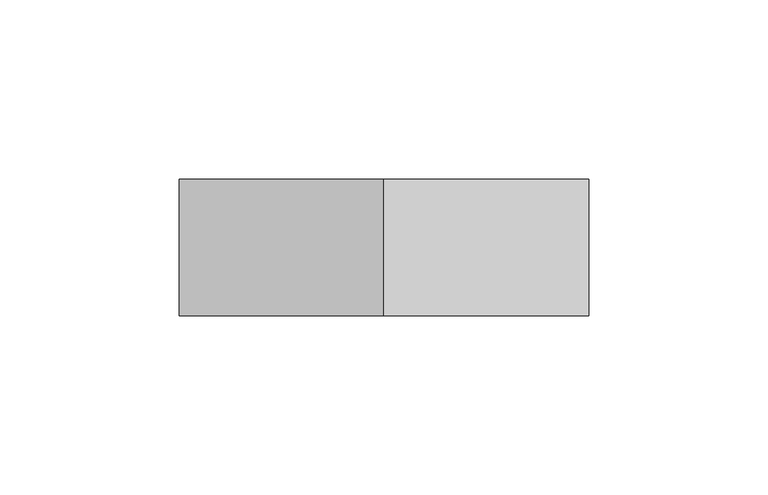
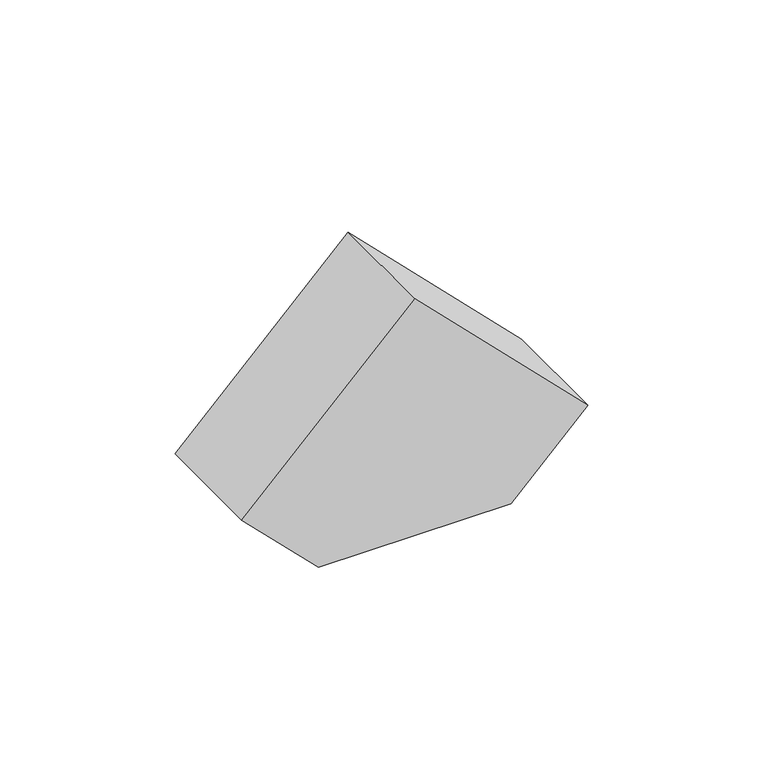
"""IFC4 building model written with IfcOpenShell, lengths in millimetres: proxy geometry, Inner panel:Inner panel:1:Inner panel:1 : Inner panel:Inner panel:300324:2:Inner panel:1:Inner panel:1 : Inner panel:Inner panel:300324:2 : Inner panel:Inner panel:1:Inner panel:1 : Inner panel:Inner panel:300324:300043:5 : Inner panel:Inner panel:1:Inner panel:1 : Inner panel:Inner panel:300324:2:Inner panel:1:Inner panel:1 : Inner panel:Inner panel:300324:2 : Inner panel:Inner panel:1:Inner panel:1 : Inner panel:Inner panel:300324:300043:308120."""

from ifc_helpers import new_model, si_unit, frame, origin, place, context, project, spatial, polyline, outline, extrude, source, transform, mapped, element, save


def generic_models_2ab5475e(model_context):
    return source(origin(), model_context, "Body", "SweptSolid", [
        extrude(outline(polyline([(8849.4498692, 566644.3220663), (8906.5998691, 566587.1720663), (8849.4498691, 566530.0220663), (8824.0498691, 566555.4220663), (8824.0498691, 566618.9220663), (8849.4498692, 566644.3220663)])), frame((0.0, -542812.2366705, 0.0), z_axis=(0.0, 1.0, 0.0), x_axis=(0.0, 0.0, 1.0)), (0.0, 0.0, 1.0), 38.1),
    ])


if __name__ == "__main__":
    model = new_model("IFC4")
    model_context = context("Model", 3, world=origin())
    ifc_project = project(units=[si_unit("LENGTHUNIT", "METRE", prefix="MILLI")], contexts=[model_context])
    site = spatial("IfcSite", under=ifc_project)
    building = spatial("IfcBuilding", under=site)
    placement = place(None, origin())
    generic_models_shape = generic_models_2ab5475e(model_context)
    element("IfcBuildingElementProxy", 1, Name="Inner panel:Inner panel:1:Inner panel:1 : Inner panel:Inner panel:300324:2:Inner panel:1:Inner panel:1 : Inner panel:Inner panel:300324:2 : Inner panel:Inner panel:1:Inner panel:1 : Inner panel:Inner panel:300324:300043:5 : Inner panel:Inner panel:1:Inner panel:1 : Inner panel:Inner panel:300324:2:Inner panel:1:Inner panel:1 : Inner panel:Inner panel:300324:2 : Inner panel:Inner panel:1:Inner panel:1 : Inner panel:Inner panel:300324:300043:308120", ObjectType="Inner panel:Inner panel:1:Inner panel:1 : Inner panel:Inner panel:300324:2:Inner panel:1:Inner panel:1 : Inner panel:Inner panel:300324:2 : Inner panel:Inner panel:1:Inner panel:1 : Inner panel:Inner panel:300324:300043:5 : Inner panel:Inner panel:1:Inner panel:1 : Inner panel:Inner panel:300324:2:Inner panel:1:Inner panel:1 : Inner panel:Inner panel:300324:2 : Inner panel:Inner panel:1:Inner panel:1 : Inner panel:Inner panel:300324:300043:308120", at=placement, inside=building, context=model_context, shape_type="MappedRepresentation", body=[
        mapped(generic_models_shape, transform((0.0, 0.0, 0.0), x_axis=(1.0, 0.0, 0.0), y_axis=(0.0, 1.0, 0.0), z_axis=(0.0, 0.0, 1.0))),
    ])
    save(model, "model.ifc")

# Revit data of these elements
# Type "Inner panel:Inner panel:1:Inner panel:1 : Inner panel:Inner panel:300324:2:Inner panel:1:Inner panel:1 : Inner panel:Inner panel:300324:2 : Inner panel:Inner panel:1:Inner panel:1 : Inner panel:Inner panel:300324:300043:5 : Inner panel:Inner panel:1:Inner panel:1 : Inner panel:Inner panel:300324:2:Inner panel:1:Inner panel:1 : Inner panel:Inner panel:300324:2 : Inner panel:Inner panel:1:Inner panel:1 : Inner panel:Inner panel:300324:300043:308120"
#   NameOverride = "Inner panel:Inner panel:1:Inner panel:1 : Inner panel:Inner panel:300324:2:Inner panel:1:Inner panel:1 : Inner panel:Inner panel:300324:2 : Inner panel:Inner panel:1:Inner panel:1 : Inner panel:Inner panel:300324:300043:308120"
#   ObjectTypeOverride = "Inner panel:1:Inner panel:1 : Inner panel:Inner panel:300324:2 : Inner panel:Inner panel:1:Inner panel:1 : Inner panel:Inner panel:300324:300043"
#   Reference = "Inner panel"
#   Tag = "308120"
# Element 1 (IfcBuildingElementProxy, "Inner panel:Inner panel:1:Inner panel:1 : Inner panel:Inner panel:300324:2:Inner panel:1:Inner panel:1 : Inner panel:Inner panel:300324:2 : Inner panel:Inner panel:1:Inner panel:1 : Inner panel:Inner panel:300324:300043:5 : Inner panel:Inner panel:1:Inner panel:1 : Inner panel:Inner panel:300324:2:Inner panel:1:Inner panel:1 : Inner panel:Inner panel:300324:2 : Inner panel:Inner panel:1:Inner panel:1 : Inner panel:Inner panel:300324:300043:308120")
#   Materials on its faces: "SNOW GUARD SYSTEM"
# Materials
#   "SNOW GUARD SYSTEM": class "Generic", colour RGB 223 223 223, transparency 0, Cost = 0
